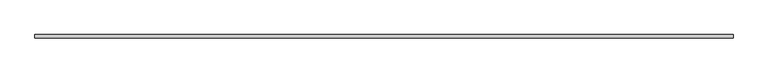
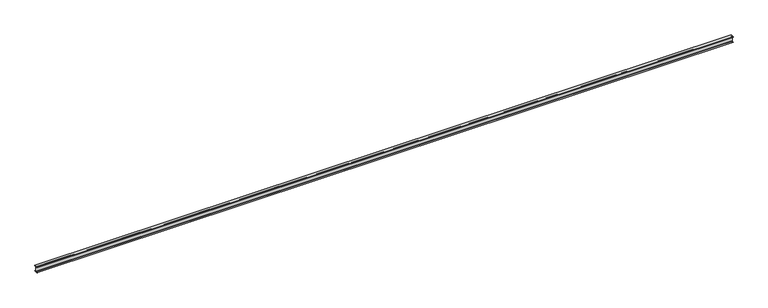
"""IFC4 building model written with IfcOpenShell, lengths in millimetres: beam geometry, Steel Framing_H_KS : H_SB_AR_S02_H-488x300x11x18_CRG1."""

from ifc_helpers import new_model, si_unit, point, frame, frame_2d, origin, place, context, project, spatial, polyline, circle_curve, trimmed, segment, composite_curve, outline, extrude, source, transform, mapped, element, save


def beam_06871935(model_context):
    return source(origin(), model_context, "Body", "SweptSolid", [
        extrude(outline(composite_curve([segment(polyline([(-150.0, -226.0), (-31.5, -226.0)]), True, "CONTINUOUS"), segment(trimmed(circle_curve(frame_2d((-31.5, -200.0)), 26.0), [point((-31.5, -226.0))], [point((-5.5, -200.0))], True, "CARTESIAN"), True, "CONTINUOUS"), segment(polyline([(-5.5, -200.0), (-5.5, 200.0)]), True, "CONTINUOUS"), segment(trimmed(circle_curve(frame_2d((-31.5, 200.0)), 26.0), [point((-5.5, 200.0))], [point((-31.5, 226.0))], True, "CARTESIAN"), True, "CONTINUOUS"), segment(polyline([(-31.5, 226.0), (-150.0, 226.0), (-150.0, 244.0), (150.0, 244.0), (150.0, 226.0), (31.5, 226.0)]), True, "CONTINUOUS"), segment(trimmed(circle_curve(frame_2d((31.5, 200.0)), 26.0), [point((31.5, 226.0))], [point((5.5, 200.0))], True, "CARTESIAN"), True, "CONTINUOUS"), segment(polyline([(5.5, 200.0), (5.5, -200.0)]), True, "CONTINUOUS"), segment(trimmed(circle_curve(frame_2d((31.5, -200.0)), 26.0), [point((5.5, -200.0))], [point((31.5, -226.0))], True, "CARTESIAN"), True, "CONTINUOUS"), segment(polyline([(31.5, -226.0), (150.0, -226.0), (150.0, -244.0), (-150.0, -244.0), (-150.0, -226.0)]), True, "CONTINUOUS")], self_intersect=False)), frame((-29987.2, 0.0, 0.0), z_axis=(1.0, 0.0, 0.0), x_axis=(0.0, 1.0, 0.0)), (0.0, 0.0, 1.0), 59974.4),
    ])


if __name__ == "__main__":
    model = new_model("IFC4")
    model_context = context("Model", 3, world=origin())
    ifc_project = project(units=[si_unit("LENGTHUNIT", "METRE", prefix="MILLI")], contexts=[model_context])
    site = spatial("IfcSite", under=ifc_project)
    building = spatial("IfcBuilding", under=site)
    placement = place(None, origin())
    beam_shape = beam_06871935(model_context)
    element("IfcBeam", 1, ObjectType="Steel Framing_H_KS : H_SB_AR_S02_H-488x300x11x18_CRG1", at=placement, inside=building, context=model_context, shape_type="MappedRepresentation", body=[
        mapped(beam_shape, transform((0.0, 0.0, 0.0), x_axis=(1.0, 0.0, 0.0), y_axis=(0.0, 1.0, 0.0), z_axis=(0.0, 0.0, 1.0))),
    ])
    save(model, "model.ifc")

# Revit data of these elements
# Type "Steel Framing_H_KS : H_SB_AR_S02_H-488x300x11x18_CRG1"
#   Type Comments = "MAIN"
#   Type Mark = "CRG1"
#   H_SectionID = "H-488x300x11x18"
#   H_Ratio for Additional Steel Plate = 0.2
#   Width = 30.0 cm
#   Web Thickness = 1.1 cm
#   Web Fillet = 2.6 cm
#   Warping Constant = 4470000.0 cm⁶
#   Torsional Moment of Inertia = 137.492 cm⁴
#   Section Area = 163.5 cm²
#   Plastic Modulus weak axis = 830.0 cm³
#   Plastic Modulus strong axis = 3230.0 cm³
#   Perimeter = 2.11 m²/m
#   Nominal Weight = 128.00 kgf/m
#   Moment of Inertia weak axis = 8110.00 cm⁴
#   Moment of Inertia strong axis = 71000.00 cm⁴
#   Height = 48.8 cm
#   Flange Thickness = 1.8 cm
#   Elastic Modulus weak axis = 541.0 cm³
#   Elastic Modulus strong axis = 2910.0 cm³
#   Centroid Vertical = 24.4 cm
#   Centroid Horizontal = 15.0 cm
#   Bolt Spacing = 8.89 cm
#   Length [instance default] = 1500 mm
#   Structural Material [instance default] = Steel, 45-345
#   Section Name Key = ""
#   Assembly Code = ""
# Element 1 (IfcBeam, "Steel Framing_H_KS : H_SB_AR_S02_H-488x300x11x18_CRG1")
#   Materials on its faces: "Steel, 45-345"
# Materials
#   "Steel, 45-345": class "Metal", colour RGB 189 187 185, transparency 0, Description = "Steel 345 MPa", Cost = 0
